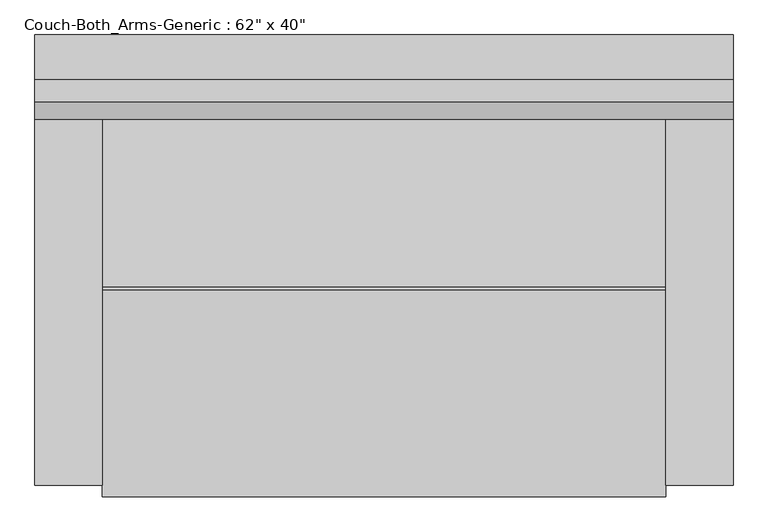
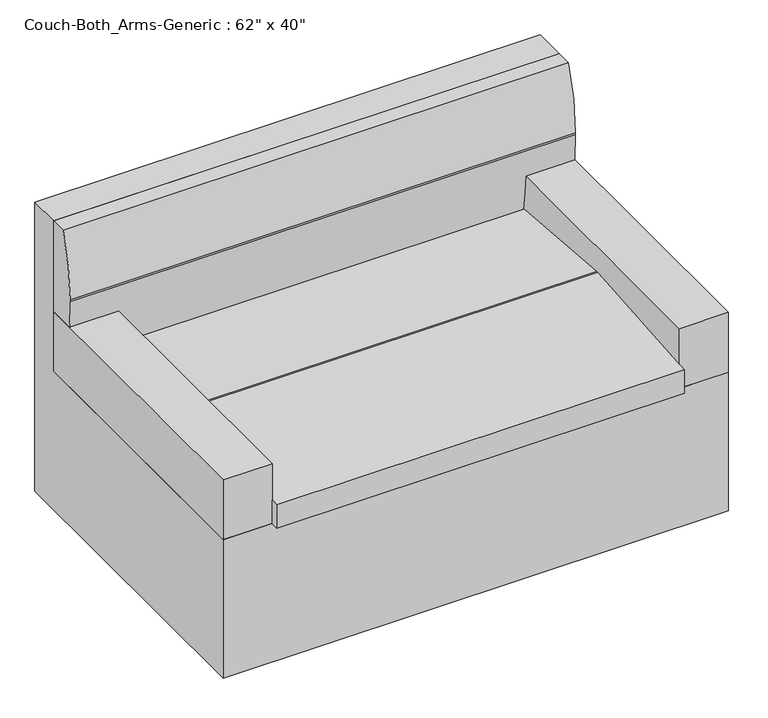
"""IFC4 building model written with IfcOpenShell, lengths in millimetres: furniture geometry."""

from ifc_helpers import new_model, si_unit, point, frame, frame_2d, origin, place, context, project, spatial, polyline, circle_curve, trimmed, segment, composite_curve, outline, extrude, source, transform, mapped, element, save
from ifc_brep_helpers import plane_surface, cylinder_surface, advanced_brep


def furniture_f8ec4437(model_context):
    return source(origin(), model_context, "Body", "SolidModel", [
        extrude(outline(composite_curve([segment(polyline([(-533.4, 457.2), (-533.4, 533.4)]), True, "CONTINUOUS"), segment(trimmed(circle_curve(frame_2d((-66.675, -2306.240625)), 2877.740625), [point((-533.4, 533.4))], [point((-66.675, 571.5))], False, "CARTESIAN"), True, "CONTINUOUS"), segment(polyline([(-66.675, 571.5), (-60.325, 571.5)]), True, "CONTINUOUS"), segment(trimmed(circle_curve(frame_2d((-60.325, -2306.240625)), 2877.740625), [point((-60.325, 571.5))], [point((406.4, 533.4))], False, "CARTESIAN"), True, "CONTINUOUS"), segment(polyline([(406.4, 533.4), (406.4, 457.2), (-533.4, 457.2)]), True, "CONTINUOUS")], self_intersect=False)), frame((-635.0, 0.0, 0.0), z_axis=(1.0, 0.0, 0.0), x_axis=(0.0, 1.0, 0.0)), (0.0, 0.0, 1.0), 1270.0),
        extrude(outline(polyline([(-635.0, 406.4), (-635.0, -508.0), (-787.4, -508.0), (-787.4, 406.4), (-635.0, 406.4)])), frame((0.0, 0.0, 457.2), z_axis=(0.0, 0.0, 1.0), x_axis=(1.0, 0.0, 0.0)), (0.0, 0.0, 1.0), 196.85),
        extrude(outline(polyline([(787.4, 406.4), (787.4, -508.0), (635.0, -508.0), (635.0, 406.4), (787.4, 406.4)])), frame((0.0, 0.0, 457.2), z_axis=(0.0, 0.0, 1.0), x_axis=(1.0, 0.0, 0.0)), (0.0, 0.0, 1.0), 196.85),
        advanced_brep(
        [(787.4, 355.6, 952.5), (787.4, 317.5, 746.125), (787.4, 317.5, 739.775), (787.4, 320.5484243, 654.05), (787.4, 406.4, 654.05), (787.4, 406.4, 952.5), (-787.4, 317.5, 739.775), (-787.4, 317.5, 746.125), (-787.4, 355.6, 952.5), (-787.4, 406.4, 952.5), (-787.4, 406.4, 654.05), (-787.4, 320.5484243, 654.05), (-635.0, 320.5484243, 654.05), (-635.0, 335.2760797, 533.4), (635.0, 335.2760797, 533.4), (635.0, 320.5484243, 654.05), (635.0, 406.4, 533.4), (-635.0, 406.4, 533.4), (635.0, 406.4, 654.05), (-635.0, 406.4, 654.05)],
        [
            (0, 1, circle_curve(frame((787.4, 895.4822917, 746.125), z_axis=(1.0, 0.0, 0.0), x_axis=(0.0, 0.0, -1.0)), 577.9822917)),
            (1, 2),
            (2, 3, circle_curve(frame((787.4, 1524.3642357, 739.775), z_axis=(1.0, 0.0, 0.0), x_axis=(0.0, 0.0, -1.0)), 1206.8642357)),
            (3, 4),
            (4, 5),
            (5, 0),
            (6, 7),
            (7, 8, circle_curve(frame((-787.4, 895.4822917, 746.125), z_axis=(-1.0, 0.0, 0.0), x_axis=(0.0, 0.0, -1.0)), 577.9822917)),
            (8, 9),
            (9, 10),
            (10, 11),
            (11, 6, circle_curve(frame((-787.4, 1524.3642357, 739.775), z_axis=(-1.0, 0.0, 0.0), x_axis=(0.0, 0.0, -1.0)), 1206.8642357)),
            (0, 8),
            (7, 1),
            (6, 2),
            (11, 12),
            (12, 13, circle_curve(frame((-635.0, 1524.3642357, 739.775), z_axis=(1.0, 0.0, 0.0), x_axis=(0.0, 0.0, -1.0)), 1206.8642357)),
            (13, 14),
            (14, 15, circle_curve(frame((635.0, 1524.3642357, 739.775), z_axis=(-1.0, 0.0, 0.0), x_axis=(0.0, 0.0, -1.0)), 1206.8642357)),
            (15, 3),
            (16, 14),
            (13, 17),
            (17, 16),
            (9, 5),
            (4, 18),
            (18, 16),
            (17, 19),
            (19, 10),
            (15, 18),
            (19, 12),
        ],
        [
            plane_surface(frame((787.4, 335.2760797, 742.95), z_axis=(1.0, 0.0, 0.0), x_axis=(0.0, -1.0, 0.0))),
            plane_surface(frame((-787.4, 335.2760797, 742.95), z_axis=(-1.0, 0.0, 0.0), x_axis=(0.0, -1.0, 0.0))),
            cylinder_surface(frame((787.4, 895.4822917, 746.125), z_axis=(1.0, 0.0, 0.0), x_axis=(0.0, 0.0, -1.0)), 577.9822917),
            plane_surface(frame((787.4, 317.5, 746.125), z_axis=(0.0, -1.0, 0.0), x_axis=(-1.0, 0.0, 0.0))),
            cylinder_surface(frame((787.4, 1524.3642357, 739.775), z_axis=(1.0, 0.0, 0.0), x_axis=(0.0, 0.0, -1.0)), 1206.8642357),
            plane_surface(frame((787.4, 335.2760797, 533.4), z_axis=(0.0, 0.0, -1.0), x_axis=(-1.0, 0.0, 0.0))),
            plane_surface(frame((-787.4, 406.4, 952.5), z_axis=(0.0, 1.0, 0.0), x_axis=(1.0, 0.0, 0.0))),
            plane_surface(frame((787.4, 355.6, 952.5), z_axis=(0.0, 0.0, 1.0), x_axis=(0.0, 1.0, 0.0))),
            plane_surface(frame((635.0, 565.15, 654.05), z_axis=(0.0, 0.0, -1.0), x_axis=(-1.0, 0.0, 0.0))),
            plane_surface(frame((635.0, 565.15, 654.05), z_axis=(1.0, 0.0, 0.0), x_axis=(0.0, 0.0, -1.0))),
            plane_surface(frame((-787.4, 514.35, 654.05), z_axis=(0.0, 0.0, -1.0), x_axis=(-1.0, 0.0, 0.0))),
            plane_surface(frame((-635.0, 165.1, 654.05), z_axis=(-1.0, 0.0, 0.0), x_axis=(0.0, 0.0, -1.0))),
        ],
        [
            (0, [[1, 2, 3, 4, 5, 6]]),
            (1, [[7, 8, 9, 10, 11, 12]]),
            (2, [[-1, 13, -8, 14]]),
            (3, [[-2, -14, -7, 15]]),
            (4, [[-15, -12, 16, 17, 18, 19, 20, -3]]),
            (5, [[21, -18, 22, 23]]),
            (6, [[24, -5, 25, 26, -23, 27, 28, -10]]),
            (7, [[-24, -9, -13, -6]]),
            (8, [[29, -25, -4, -20]]),
            (9, [[-29, -19, -21, -26]]),
            (10, [[30, -16, -11, -28]]),
            (11, [[-30, -27, -22, -17]]),
        ],
    ),
        extrude(outline(polyline([(-508.0, 457.2), (406.4, 457.2), (406.4, 952.5), (508.0, 952.5), (508.0, 0.0), (-508.0, 0.0), (-508.0, 457.2)])), frame((-787.4, 0.0, 0.0), z_axis=(1.0, 0.0, 0.0), x_axis=(0.0, 1.0, 0.0)), (0.0, 0.0, 1.0), 1574.8),
    ])


if __name__ == "__main__":
    model = new_model("IFC4")
    model_context = context("Model", 3, world=origin())
    ifc_project = project(units=[si_unit("LENGTHUNIT", "METRE", prefix="MILLI")], contexts=[model_context])
    site = spatial("IfcSite", under=ifc_project)
    building = spatial("IfcBuilding", under=site)
    placement = place(None, origin())
    furniture_shape = furniture_f8ec4437(model_context)
    element("IfcFurniture", 1, ObjectType="Couch-Both_Arms-Generic : 62\" x 40\"", at=placement, inside=building, context=model_context, shape_type="MappedRepresentation", body=[
        mapped(furniture_shape, transform((0.0, 0.0, 0.0), x_axis=(1.0, 0.0, 0.0), y_axis=(0.0, 1.0, 0.0), z_axis=(0.0, 0.0, 1.0))),
    ])
    save(model, "model.ifc")

# Revit data of these elements
# Type "Couch-Both_Arms-Generic : 62\" x 40\""
#   OmniClass Title = "Settees, Sofas"
#   OmniClass Number = "23.40.20.14.14.14"
#   Model = "Both Arms"
#   Manufacturer = "Generic"
#   Description = "Straight Couch with armrests on both sides"
#   Width = 5' - 2"
#   Seat Height = 1' - 6"
#   Height = 3' - 1 1/2"
#   Depth = 3' - 4"
#   Couch Cushion Width = 4' - 2"
#   Couch Cushion Depth = 3' - 1"
#   Backseat Height = 1' - 4 1/2"
#   Arm Rest Width = 0' - 6"
#   Arm Rest Depth = 3' - 0"
#   Surface Finish = none
#   Type Comments = ""
#   Keynote = ""
#   Assembly Code = ""
